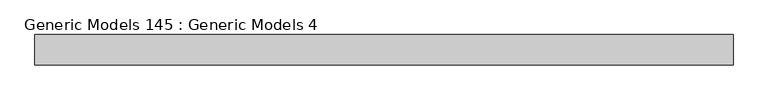
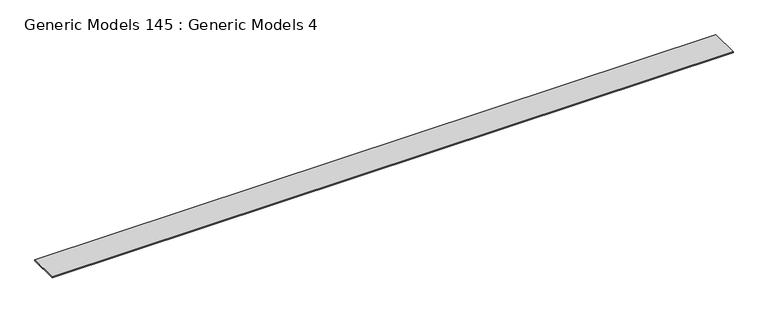
"""IFC4 building model written with IfcOpenShell, lengths in millimetres: proxy geometry, Generic Models 145 : Generic Models 4."""

import ifcopenshell
import ifcopenshell.guid

model = None  # the IFC model being written
_history = None  # IfcOwnerHistory: only IFC2X3 demands one
_inside = {}  # id of a spatial element -> (the spatial element, [elements in it])
_under = {}  # id of a project, library or spatial element -> (it, [spatial elements below it])
_declared = {}  # id of a project -> (the project, [libraries it declares])
_typed = {}  # id of a type object -> (the type object, [elements of that type])
_made_of = {}  # id of a material, layer set ... -> (it, [elements and type objects made of it])


def new_model(schema):
    """Start an empty IFC model of exactly this schema.

    Asked for "IFC4X3", IfcOpenShell would pick the latest addendum, in which some entities
    have other attributes; the version numbers below select the first issue.
    IFC2X3 requires an IfcOwnerHistory on every rooted entity: one is made here for all.
    """
    global model, _history
    if schema == "IFC4X3":
        model = ifcopenshell.file(schema_version=(4, 3, 0, 0))
    else:
        model = ifcopenshell.file(schema=schema)
    _inside.clear()
    _under.clear()
    _declared.clear()
    _typed.clear()
    _made_of.clear()
    _history = None
    if model.schema == "IFC2X3":
        org = make("IfcOrganization", Name="unknown")
        user = make(
            "IfcPersonAndOrganization",
            ThePerson=make("IfcPerson", FamilyName="unknown"),
            TheOrganization=org,
        )
        app = make(
            "IfcApplication",
            ApplicationDeveloper=org,
            Version="unknown",
            ApplicationFullName="unknown",
            ApplicationIdentifier="unknown",
        )
        _history = make(
            "IfcOwnerHistory",
            OwningUser=user,
            OwningApplication=app,
            ChangeAction="ADDED",
            CreationDate=0,
        )
    return model


def make(cls, **values):
    """One entity of the class cls with the attributes given. An attribute that is None is left unset."""
    return model.create_entity(
        cls, **{name: value for name, value in values.items() if value is not None}
    )


def rooted(cls, **values):
    """An entity with a GlobalId (a new one), such as an element, a storey or a relation."""
    return make(cls, GlobalId=ifcopenshell.guid.new(), OwnerHistory=_history, **values)


def si_unit(unit_type, name, prefix=None):
    """IfcSIUnit, for example si_unit("LENGTHUNIT", "METRE", prefix="MILLI")."""
    return make("IfcSIUnit", UnitType=unit_type, Prefix=prefix, Name=name)


def assignment(units):
    """IfcUnitAssignment: the units of a project."""
    return None if units is None else make("IfcUnitAssignment", Units=units)


def point(xyz):
    """IfcCartesianPoint."""
    return None if xyz is None else make("IfcCartesianPoint", Coordinates=xyz)


def direction(xyz):
    """IfcDirection."""
    return None if xyz is None else make("IfcDirection", DirectionRatios=xyz)


def frame(location, z_axis=None, x_axis=None):
    """IfcAxis2Placement3D, a coordinate frame: its origin and axes. An axis left out is left unset."""
    return make(
        "IfcAxis2Placement3D",
        Location=point(location),
        Axis=direction(z_axis),
        RefDirection=direction(x_axis),
    )


def origin():
    """The frame at (0, 0, 0) with its axes left unset."""
    return frame((0.0, 0.0, 0.0))


def place(relative_to, where):
    """IfcLocalPlacement: puts the frame where relative to a parent placement (None: the world)."""
    return make(
        "IfcLocalPlacement", PlacementRelTo=relative_to, RelativePlacement=where
    )


def context(
    kind, dimensions, precision=None, world=None, true_north=None, identifier=None
):
    """IfcGeometricRepresentationContext, for example the 3D "Model" context."""
    return make(
        "IfcGeometricRepresentationContext",
        ContextIdentifier=identifier,
        ContextType=kind,
        CoordinateSpaceDimension=dimensions,
        Precision=precision,
        WorldCoordinateSystem=world,
        TrueNorth=true_north,
    )


def project(units=None, contexts=None):
    """IfcProject with its units and contexts."""
    return rooted(
        "IfcProject",
        Name="project",
        RepresentationContexts=contexts,
        UnitsInContext=assignment(units),
    )


def spatial(cls, under=None, at=None, **own):
    """A site, building, storey or space (cls), placed at a placement, below another one or the project."""
    s = rooted(cls, ObjectPlacement=at, **own)
    if under is not None:
        _under.setdefault(under.id(), (under, []))[1].append(s)
    return s


def polyline(points):
    """IfcPolyline through the points."""
    return make("IfcPolyline", Points=[point(p) for p in points])


def outline(outer, holes=None, kind="AREA"):
    """IfcArbitraryClosedProfileDef: a profile drawn as a closed curve; with holes, ...WithVoids."""
    if holes is None:
        return make("IfcArbitraryClosedProfileDef", ProfileType=kind, OuterCurve=outer)
    return make(
        "IfcArbitraryProfileDefWithVoids",
        ProfileType=kind,
        OuterCurve=outer,
        InnerCurves=holes,
    )


def extrude(swept, where, along, depth):
    """IfcExtrudedAreaSolid: the profile swept, set in the frame where, extruded along a direction by depth."""
    return make(
        "IfcExtrudedAreaSolid",
        SweptArea=swept,
        Position=where,
        ExtrudedDirection=direction(along),
        Depth=depth,
    )


def shape(context_of_items, identifier, shape_type, items):
    """IfcShapeRepresentation: the items that make up one representation, for example the "Body"."""
    return make(
        "IfcShapeRepresentation",
        ContextOfItems=context_of_items,
        RepresentationIdentifier=identifier,
        RepresentationType=shape_type,
        Items=items,
    )


def source(mapping_origin, context_of_items, identifier, shape_type, items):
    """IfcRepresentationMap: a shape defined once, which mapped items show again and again."""
    return make(
        "IfcRepresentationMap",
        MappingOrigin=mapping_origin,
        MappedRepresentation=shape(context_of_items, identifier, shape_type, items),
    )


def transform(
    local_origin,
    x_axis=None,
    y_axis=None,
    z_axis=None,
    scale=None,
    scale2=None,
    scale3=None,
    uniform=True,
):
    """IfcCartesianTransformationOperator3D, or its non-uniform kind. x_axis, y_axis, z_axis: its Axis1, 2, 3."""
    if uniform:
        return make(
            "IfcCartesianTransformationOperator3D",
            Axis1=direction(x_axis),
            Axis2=direction(y_axis),
            LocalOrigin=point(local_origin),
            Scale=scale,
            Axis3=direction(z_axis),
        )
    return make(
        "IfcCartesianTransformationOperator3DnonUniform",
        Axis1=direction(x_axis),
        Axis2=direction(y_axis),
        LocalOrigin=point(local_origin),
        Scale=scale,
        Axis3=direction(z_axis),
        Scale2=scale2,
        Scale3=scale3,
    )


def mapped(mapping_source, mapping_target):
    """IfcMappedItem: shows the shape of a source again, moved by a transform."""
    return make(
        "IfcMappedItem", MappingSource=mapping_source, MappingTarget=mapping_target
    )


def made_of(thing, what):
    """Note that an element or type object is made of a material, layer set ...; save() writes the relation."""
    if what is not None:
        _made_of.setdefault(what.id(), (what, []))[1].append(thing)
    return thing


def element(
    cls,
    number,
    at=None,
    inside=None,
    cuts=None,
    type_object=None,
    material=None,
    context=None,
    identifier="Body",
    shape_type=None,
    held_by="IfcProductDefinitionShape",
    body=None,
    shapes=None,
    **own,
):
    """One element of the class cls, such as IfcWall. Its Tag is "e" and its number.

    at: its placement. inside: the storey or other place that contains it. cuts: it is an
    opening in that element (IfcRelVoidsElement). A single representation is given by context,
    identifier, shape_type and body (its items); several are given by shapes. held_by: the class
    of the entity that holds the representations. save() writes the other relations.
    """
    e = rooted(cls, Tag="e%d" % number, ObjectPlacement=at, **own)
    if body is not None:
        shapes = [shape(context, identifier, shape_type, body)]
    if shapes is not None:
        e.Representation = make(held_by, Representations=shapes)
    if inside is not None:
        _inside.setdefault(inside.id(), (inside, []))[1].append(e)
    if cuts is not None:
        rooted(
            "IfcRelVoidsElement", RelatingBuildingElement=cuts, RelatedOpeningElement=e
        )
    if type_object is not None:
        _typed.setdefault(type_object.id(), (type_object, []))[1].append(e)
    return made_of(e, material)


def aggregate(whole, parts):
    """IfcRelAggregates: a whole, such as a stair, and the parts it consists of."""
    return rooted("IfcRelAggregates", RelatingObject=whole, RelatedObjects=parts)


def save(model, path):
    """Write the relations noted so far, then the file.

    IfcRelAggregates (storeys below a building ...), IfcRelContainedInSpatialStructure (elements
    in a storey), IfcRelDefinesByType, IfcRelAssociatesMaterial and IfcRelDeclares: one each for
    every whole, place, type object, material and project.
    """
    for whole, parts in _under.values():
        aggregate(whole, parts)
    for where, things in _inside.values():
        rooted(
            "IfcRelContainedInSpatialStructure",
            RelatedElements=things,
            RelatingStructure=where,
        )
    for kind, things in _typed.values():
        rooted("IfcRelDefinesByType", RelatedObjects=things, RelatingType=kind)
    for what, things in _made_of.values():
        rooted("IfcRelAssociatesMaterial", RelatedObjects=things, RelatingMaterial=what)
    for by, libraries in _declared.values():
        rooted("IfcRelDeclares", RelatingContext=by, RelatedDefinitions=libraries)
    model.write(path)


def generic_models_145_generic_models_4_e898942e(model_context):
    return source(origin(), model_context, "Body", "SweptSolid", [
        extrude(outline(polyline([(-19489.9914237, 7053.8569221), (-19489.9914237, 7602.3455867), (-6942.3914237, 7602.3455867), (-6942.3914237, 7053.8569221), (-19489.9914237, 7053.8569221)])), frame((0.0, 0.0, 123443.746), z_axis=(0.0, 0.0, 1.0), x_axis=(1.0, 0.0, 0.0)), (0.0, 0.0, 1.0), 19.05),
    ])


if __name__ == "__main__":
    model = new_model("IFC4")
    model_context = context("Model", 3, world=origin())
    ifc_project = project(units=[si_unit("LENGTHUNIT", "METRE", prefix="MILLI")], contexts=[model_context])
    site = spatial("IfcSite", under=ifc_project)
    building = spatial("IfcBuilding", under=site)
    placement = place(None, origin())
    generic_models_145_generic_models_4_shape = generic_models_145_generic_models_4_e898942e(model_context)
    element("IfcBuildingElementProxy", 1, Name="Generic Models 145 : Generic Models 4", ObjectType="Generic Models 145 : Generic Models 4", at=placement, inside=building, context=model_context, shape_type="MappedRepresentation", body=[
        mapped(generic_models_145_generic_models_4_shape, transform((0.0, 0.0, 0.0), x_axis=(1.0, 0.0, 0.0), y_axis=(0.0, 1.0, 0.0), z_axis=(0.0, 0.0, 1.0))),
    ])
    save(model, "model.ifc")

# Revit data of these elements
# Element 1 (IfcBuildingElementProxy, "Generic Models 145 : Generic Models 4")
#   Materials on its faces: "_WOOD FLOORING (SPEC T.B.D.)"
# Materials
#   "_WOOD FLOORING (SPEC T.B.D.)": class "Generic", colour RGB 177 130 114, transparency 0, Cost = 0
